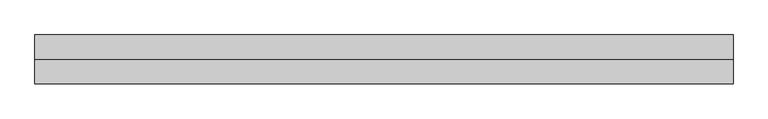
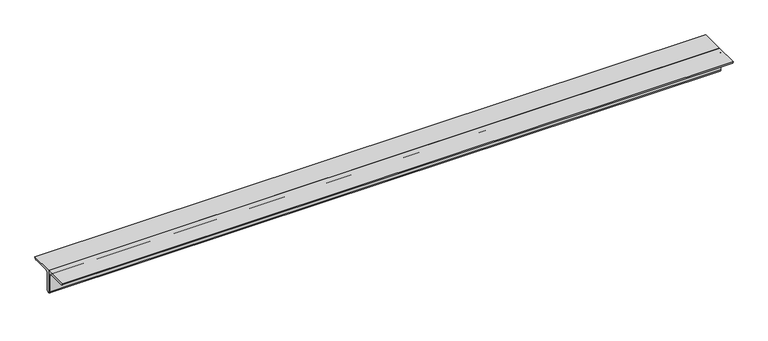
"""IFC4 building model written with IfcOpenShell, lengths in millimetres: member geometry, 0123_Steel Framing_2Ls-KSD3502 : H_SB_AR_S03_2Ls-130x130x12_HBR1."""

import ifcopenshell
import ifcopenshell.guid

model = None  # the IFC model being written
_history = None  # IfcOwnerHistory: only IFC2X3 demands one
_inside = {}  # id of a spatial element -> (the spatial element, [elements in it])
_under = {}  # id of a project, library or spatial element -> (it, [spatial elements below it])
_declared = {}  # id of a project -> (the project, [libraries it declares])
_typed = {}  # id of a type object -> (the type object, [elements of that type])
_made_of = {}  # id of a material, layer set ... -> (it, [elements and type objects made of it])


def new_model(schema):
    """Start an empty IFC model of exactly this schema.

    Asked for "IFC4X3", IfcOpenShell would pick the latest addendum, in which some entities
    have other attributes; the version numbers below select the first issue.
    IFC2X3 requires an IfcOwnerHistory on every rooted entity: one is made here for all.
    """
    global model, _history
    if schema == "IFC4X3":
        model = ifcopenshell.file(schema_version=(4, 3, 0, 0))
    else:
        model = ifcopenshell.file(schema=schema)
    _inside.clear()
    _under.clear()
    _declared.clear()
    _typed.clear()
    _made_of.clear()
    _history = None
    if model.schema == "IFC2X3":
        org = make("IfcOrganization", Name="unknown")
        user = make(
            "IfcPersonAndOrganization",
            ThePerson=make("IfcPerson", FamilyName="unknown"),
            TheOrganization=org,
        )
        app = make(
            "IfcApplication",
            ApplicationDeveloper=org,
            Version="unknown",
            ApplicationFullName="unknown",
            ApplicationIdentifier="unknown",
        )
        _history = make(
            "IfcOwnerHistory",
            OwningUser=user,
            OwningApplication=app,
            ChangeAction="ADDED",
            CreationDate=0,
        )
    return model


def make(cls, **values):
    """One entity of the class cls with the attributes given. An attribute that is None is left unset."""
    return model.create_entity(
        cls, **{name: value for name, value in values.items() if value is not None}
    )


def rooted(cls, **values):
    """An entity with a GlobalId (a new one), such as an element, a storey or a relation."""
    return make(cls, GlobalId=ifcopenshell.guid.new(), OwnerHistory=_history, **values)


def si_unit(unit_type, name, prefix=None):
    """IfcSIUnit, for example si_unit("LENGTHUNIT", "METRE", prefix="MILLI")."""
    return make("IfcSIUnit", UnitType=unit_type, Prefix=prefix, Name=name)


def assignment(units):
    """IfcUnitAssignment: the units of a project."""
    return None if units is None else make("IfcUnitAssignment", Units=units)


def point(xyz):
    """IfcCartesianPoint."""
    return None if xyz is None else make("IfcCartesianPoint", Coordinates=xyz)


def direction(xyz):
    """IfcDirection."""
    return None if xyz is None else make("IfcDirection", DirectionRatios=xyz)


def frame(location, z_axis=None, x_axis=None):
    """IfcAxis2Placement3D, a coordinate frame: its origin and axes. An axis left out is left unset."""
    return make(
        "IfcAxis2Placement3D",
        Location=point(location),
        Axis=direction(z_axis),
        RefDirection=direction(x_axis),
    )


def frame_2d(location, x_axis=None):
    """IfcAxis2Placement2D, a coordinate frame in the plane: its origin and x axis."""
    return make(
        "IfcAxis2Placement2D", Location=point(location), RefDirection=direction(x_axis)
    )


def origin():
    """The frame at (0, 0, 0) with its axes left unset."""
    return frame((0.0, 0.0, 0.0))


def place(relative_to, where):
    """IfcLocalPlacement: puts the frame where relative to a parent placement (None: the world)."""
    return make(
        "IfcLocalPlacement", PlacementRelTo=relative_to, RelativePlacement=where
    )


def context(
    kind, dimensions, precision=None, world=None, true_north=None, identifier=None
):
    """IfcGeometricRepresentationContext, for example the 3D "Model" context."""
    return make(
        "IfcGeometricRepresentationContext",
        ContextIdentifier=identifier,
        ContextType=kind,
        CoordinateSpaceDimension=dimensions,
        Precision=precision,
        WorldCoordinateSystem=world,
        TrueNorth=true_north,
    )


def project(units=None, contexts=None):
    """IfcProject with its units and contexts."""
    return rooted(
        "IfcProject",
        Name="project",
        RepresentationContexts=contexts,
        UnitsInContext=assignment(units),
    )


def spatial(cls, under=None, at=None, **own):
    """A site, building, storey or space (cls), placed at a placement, below another one or the project."""
    s = rooted(cls, ObjectPlacement=at, **own)
    if under is not None:
        _under.setdefault(under.id(), (under, []))[1].append(s)
    return s


def polyline(points):
    """IfcPolyline through the points."""
    return make("IfcPolyline", Points=[point(p) for p in points])


def circle_curve(where, radius):
    """IfcCircle in the frame where."""
    return make("IfcCircle", Position=where, Radius=radius)


def trimmed(basis, trim1, trim2, sense, master):
    """IfcTrimmedCurve: the piece of a basis curve between two trims."""
    return make(
        "IfcTrimmedCurve",
        BasisCurve=basis,
        Trim1=trim1,
        Trim2=trim2,
        SenseAgreement=sense,
        MasterRepresentation=master,
    )


def segment(curve, same_sense, transition):
    """IfcCompositeCurveSegment."""
    return make(
        "IfcCompositeCurveSegment",
        Transition=transition,
        SameSense=same_sense,
        ParentCurve=curve,
    )


def composite_curve(segments, self_intersect=None):
    """IfcCompositeCurve: segments joined end to end."""
    return make("IfcCompositeCurve", Segments=segments, SelfIntersect=self_intersect)


def outline(outer, holes=None, kind="AREA"):
    """IfcArbitraryClosedProfileDef: a profile drawn as a closed curve; with holes, ...WithVoids."""
    if holes is None:
        return make("IfcArbitraryClosedProfileDef", ProfileType=kind, OuterCurve=outer)
    return make(
        "IfcArbitraryProfileDefWithVoids",
        ProfileType=kind,
        OuterCurve=outer,
        InnerCurves=holes,
    )


def extrude(swept, where, along, depth):
    """IfcExtrudedAreaSolid: the profile swept, set in the frame where, extruded along a direction by depth."""
    return make(
        "IfcExtrudedAreaSolid",
        SweptArea=swept,
        Position=where,
        ExtrudedDirection=direction(along),
        Depth=depth,
    )


def shape(context_of_items, identifier, shape_type, items):
    """IfcShapeRepresentation: the items that make up one representation, for example the "Body"."""
    return make(
        "IfcShapeRepresentation",
        ContextOfItems=context_of_items,
        RepresentationIdentifier=identifier,
        RepresentationType=shape_type,
        Items=items,
    )


def source(mapping_origin, context_of_items, identifier, shape_type, items):
    """IfcRepresentationMap: a shape defined once, which mapped items show again and again."""
    return make(
        "IfcRepresentationMap",
        MappingOrigin=mapping_origin,
        MappedRepresentation=shape(context_of_items, identifier, shape_type, items),
    )


def transform(
    local_origin,
    x_axis=None,
    y_axis=None,
    z_axis=None,
    scale=None,
    scale2=None,
    scale3=None,
    uniform=True,
):
    """IfcCartesianTransformationOperator3D, or its non-uniform kind. x_axis, y_axis, z_axis: its Axis1, 2, 3."""
    if uniform:
        return make(
            "IfcCartesianTransformationOperator3D",
            Axis1=direction(x_axis),
            Axis2=direction(y_axis),
            LocalOrigin=point(local_origin),
            Scale=scale,
            Axis3=direction(z_axis),
        )
    return make(
        "IfcCartesianTransformationOperator3DnonUniform",
        Axis1=direction(x_axis),
        Axis2=direction(y_axis),
        LocalOrigin=point(local_origin),
        Scale=scale,
        Axis3=direction(z_axis),
        Scale2=scale2,
        Scale3=scale3,
    )


def mapped(mapping_source, mapping_target):
    """IfcMappedItem: shows the shape of a source again, moved by a transform."""
    return make(
        "IfcMappedItem", MappingSource=mapping_source, MappingTarget=mapping_target
    )


def made_of(thing, what):
    """Note that an element or type object is made of a material, layer set ...; save() writes the relation."""
    if what is not None:
        _made_of.setdefault(what.id(), (what, []))[1].append(thing)
    return thing


def element(
    cls,
    number,
    at=None,
    inside=None,
    cuts=None,
    type_object=None,
    material=None,
    context=None,
    identifier="Body",
    shape_type=None,
    held_by="IfcProductDefinitionShape",
    body=None,
    shapes=None,
    **own,
):
    """One element of the class cls, such as IfcWall. Its Tag is "e" and its number.

    at: its placement. inside: the storey or other place that contains it. cuts: it is an
    opening in that element (IfcRelVoidsElement). A single representation is given by context,
    identifier, shape_type and body (its items); several are given by shapes. held_by: the class
    of the entity that holds the representations. save() writes the other relations.
    """
    e = rooted(cls, Tag="e%d" % number, ObjectPlacement=at, **own)
    if body is not None:
        shapes = [shape(context, identifier, shape_type, body)]
    if shapes is not None:
        e.Representation = make(held_by, Representations=shapes)
    if inside is not None:
        _inside.setdefault(inside.id(), (inside, []))[1].append(e)
    if cuts is not None:
        rooted(
            "IfcRelVoidsElement", RelatingBuildingElement=cuts, RelatedOpeningElement=e
        )
    if type_object is not None:
        _typed.setdefault(type_object.id(), (type_object, []))[1].append(e)
    return made_of(e, material)


def aggregate(whole, parts):
    """IfcRelAggregates: a whole, such as a stair, and the parts it consists of."""
    return rooted("IfcRelAggregates", RelatingObject=whole, RelatedObjects=parts)


def save(model, path):
    """Write the relations noted so far, then the file.

    IfcRelAggregates (storeys below a building ...), IfcRelContainedInSpatialStructure (elements
    in a storey), IfcRelDefinesByType, IfcRelAssociatesMaterial and IfcRelDeclares: one each for
    every whole, place, type object, material and project.
    """
    for whole, parts in _under.values():
        aggregate(whole, parts)
    for where, things in _inside.values():
        rooted(
            "IfcRelContainedInSpatialStructure",
            RelatedElements=things,
            RelatingStructure=where,
        )
    for kind, things in _typed.values():
        rooted("IfcRelDefinesByType", RelatedObjects=things, RelatingType=kind)
    for what, things in _made_of.values():
        rooted("IfcRelAssociatesMaterial", RelatedObjects=things, RelatingMaterial=what)
    for by, libraries in _declared.values():
        rooted("IfcRelDeclares", RelatingContext=by, RelatedDefinitions=libraries)
    model.write(path)


def member_1f5b8c5a(model_context):
    return source(origin(), model_context, "Body", "SweptSolid", [
        extrude(outline(composite_curve([segment(polyline([(0.0, 36.4), (130.0, 36.4)]), True, "CONTINUOUS"), segment(trimmed(circle_curve(frame_2d((118.0, 36.4)), 12.0), [point((130.0, 36.4))], [point((118.0, 24.4))], False, "CARTESIAN"), True, "CONTINUOUS"), segment(polyline([(118.0, 24.4), (24.0, 24.4)]), True, "CONTINUOUS"), segment(trimmed(circle_curve(frame_2d((24.0, 12.4)), 12.0), [point((24.0, 24.4))], [point((12.0, 12.4))], True, "CARTESIAN"), True, "CONTINUOUS"), segment(polyline([(12.0, 12.4), (12.0, -81.6)]), True, "CONTINUOUS"), segment(trimmed(circle_curve(frame_2d((0.0, -81.6)), 12.0), [point((12.0, -81.6))], [point((0.0, -93.6))], False, "CARTESIAN"), True, "CONTINUOUS"), segment(polyline([(0.0, -93.6), (0.0, 36.4)]), True, "CONTINUOUS")], self_intersect=False)), frame((-1844.6975967, 0.0, 0.0), z_axis=(1.0, 0.0, 0.0), x_axis=(0.0, 1.0, 0.0)), (0.0, 0.0, 1.0), 3701.6272171),
        extrude(outline(composite_curve([segment(polyline([(0.0, 36.4), (0.0, -93.6)]), True, "CONTINUOUS"), segment(trimmed(circle_curve(frame_2d((0.0, -81.6)), 12.0), [point((0.0, -93.6))], [point((-12.0, -81.6))], False, "CARTESIAN"), True, "CONTINUOUS"), segment(polyline([(-12.0, -81.6), (-12.0, 12.4)]), True, "CONTINUOUS"), segment(trimmed(circle_curve(frame_2d((-24.0, 12.4)), 12.0), [point((-12.0, 12.4))], [point((-24.0, 24.4))], True, "CARTESIAN"), True, "CONTINUOUS"), segment(polyline([(-24.0, 24.4), (-118.0, 24.4)]), True, "CONTINUOUS"), segment(trimmed(circle_curve(frame_2d((-118.0, 36.4)), 12.0), [point((-118.0, 24.4))], [point((-130.0, 36.4))], False, "CARTESIAN"), True, "CONTINUOUS"), segment(polyline([(-130.0, 36.4), (0.0, 36.4)]), True, "CONTINUOUS")], self_intersect=False)), frame((-1844.6975967, 0.0, 0.0), z_axis=(1.0, 0.0, 0.0), x_axis=(0.0, 1.0, 0.0)), (0.0, 0.0, 1.0), 3701.6272171),
    ])


if __name__ == "__main__":
    model = new_model("IFC4")
    model_context = context("Model", 3, world=origin())
    ifc_project = project(units=[si_unit("LENGTHUNIT", "METRE", prefix="MILLI")], contexts=[model_context])
    site = spatial("IfcSite", under=ifc_project)
    building = spatial("IfcBuilding", under=site)
    placement = place(None, origin())
    member_shape = member_1f5b8c5a(model_context)
    element("IfcMember", 1, ObjectType="0123_Steel Framing_2Ls-KSD3502 : H_SB_AR_S03_2Ls-130x130x12_HBR1", at=placement, inside=building, context=model_context, shape_type="MappedRepresentation", body=[
        mapped(member_shape, transform((0.0, 0.0, 0.0), x_axis=(1.0, 0.0, 0.0), y_axis=(0.0, 1.0, 0.0), z_axis=(0.0, 0.0, 1.0))),
    ])
    save(model, "model.ifc")

# Revit data of these elements
# Type "0123_Steel Framing_2Ls-KSD3502 : H_SB_AR_S03_2Ls-130x130x12_HBR1"
#   Type Mark = "HBR1"
#   Assembly Code = "B10"
#   Legs = "SLBB"
#   W = 8.97
#   Perimeter = 1.04 m²/m
#   Nominal Weight = 46.80 kgf/m
#   Length [instance default] = 1000 mm
#   Space = 0 mm
#   b = 130 mm
#   d = 130 mm
#   t = 12 mm
#   y = 36.4 mm
#   A = 0.005952 m²
#   Structural Material [instance default] = Steel ASTM A36
# Element 1 (IfcMember, "0123_Steel Framing_2Ls-KSD3502 : H_SB_AR_S03_2Ls-130x130x12_HBR1")
#   Materials on its faces: "Steel ASTM A36"
# Materials
#   "Steel ASTM A36": class "Metal", colour RGB 199 199 199, transparency 0, Description = "Structural steel, ASTM A36 Grade B, mill finish", Cost = 0
